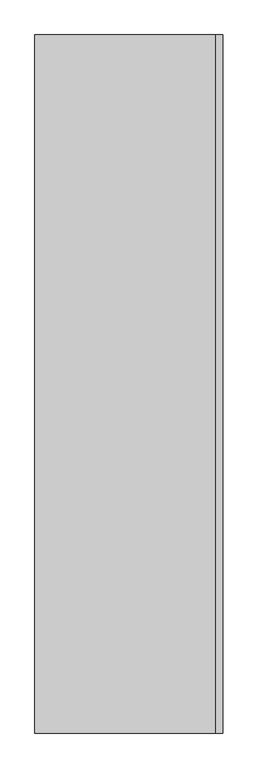
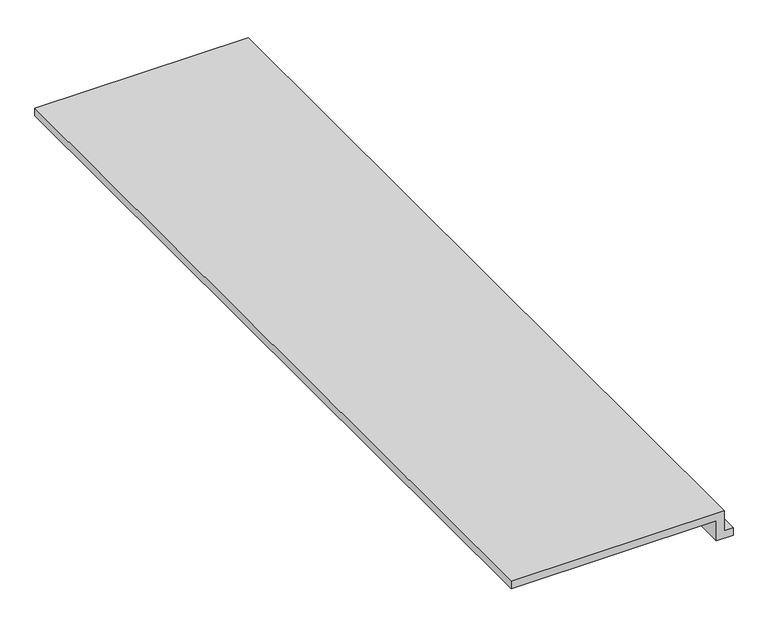
"""IFC4 building model written with IfcOpenShell, lengths in millimetres: proxy geometry, Gypsum026 11309 : Gypsum026 11309."""

from ifc_helpers import new_model, si_unit, frame, origin, place, context, project, spatial, polyline, outline, extrude, source, transform, mapped, element, save


def generic_models_0701cc7d(model_context):
    return source(origin(), model_context, "Body", "SweptSolid", [
        extrude(outline(polyline([(43005.4089179, 16509.2543635), (43056.2089179, 16509.2543635), (43056.2089179, 15992.0976563), (43037.1589179, 15992.0976563), (43037.1589179, 16490.2043635), (42986.3589179, 16490.2043635), (42986.3589179, 16530.6464844), (43005.4089179, 16530.6464844), (43005.4089179, 16509.2543635)])), frame((0.0, 7982.1435508, 0.0), z_axis=(0.0, 1.0, 0.0), x_axis=(0.0, 0.0, 1.0)), (0.0, 0.0, 1.0), 2000.0),
    ])


if __name__ == "__main__":
    model = new_model("IFC4")
    model_context = context("Model", 3, world=origin())
    ifc_project = project(units=[si_unit("LENGTHUNIT", "METRE", prefix="MILLI")], contexts=[model_context])
    site = spatial("IfcSite", under=ifc_project)
    building = spatial("IfcBuilding", under=site)
    placement = place(None, origin())
    generic_models_shape = generic_models_0701cc7d(model_context)
    element("IfcBuildingElementProxy", 1, Name="Gypsum026 11309 : Gypsum026 11309", ObjectType="Gypsum026 11309 : Gypsum026 11309", at=placement, inside=building, context=model_context, shape_type="MappedRepresentation", body=[
        mapped(generic_models_shape, transform((0.0, 0.0, 0.0), x_axis=(1.0, 0.0, 0.0), y_axis=(0.0, 1.0, 0.0), z_axis=(0.0, 0.0, 1.0))),
    ])
    save(model, "model.ifc")

# Revit data of these elements
# Type "Gypsum026 11309 : Gypsum026 11309"
#   NameOverride = "Gypsum026"
# Element 1 (IfcBuildingElementProxy, "Gypsum026 11309 : Gypsum026 11309")
#   Materials on its faces: "5/8\" GYPSUM BOARD"
# Materials
#   "5/8\" GYPSUM BOARD": class "Unassigned", colour RGB 255 255 255, transparency 0, Cost = 0
